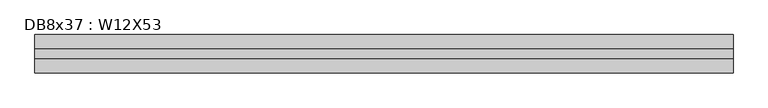
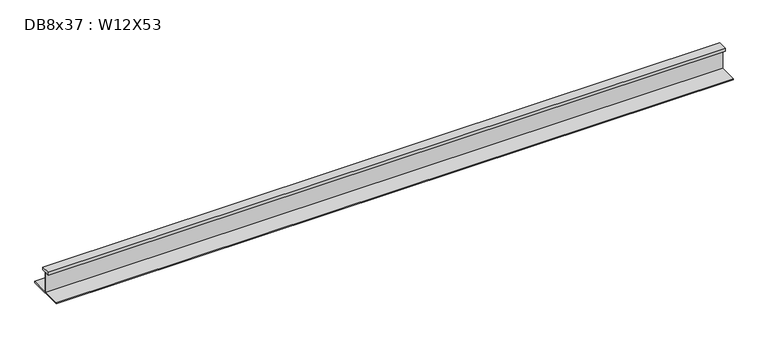
"""IFC4 building model written with IfcOpenShell, lengths in millimetres: beam geometry, DB8x37 : W12X53."""

import ifcopenshell
import ifcopenshell.guid

model = None  # the IFC model being written
_history = None  # IfcOwnerHistory: only IFC2X3 demands one
_inside = {}  # id of a spatial element -> (the spatial element, [elements in it])
_under = {}  # id of a project, library or spatial element -> (it, [spatial elements below it])
_declared = {}  # id of a project -> (the project, [libraries it declares])
_typed = {}  # id of a type object -> (the type object, [elements of that type])
_made_of = {}  # id of a material, layer set ... -> (it, [elements and type objects made of it])


def new_model(schema):
    """Start an empty IFC model of exactly this schema.

    Asked for "IFC4X3", IfcOpenShell would pick the latest addendum, in which some entities
    have other attributes; the version numbers below select the first issue.
    IFC2X3 requires an IfcOwnerHistory on every rooted entity: one is made here for all.
    """
    global model, _history
    if schema == "IFC4X3":
        model = ifcopenshell.file(schema_version=(4, 3, 0, 0))
    else:
        model = ifcopenshell.file(schema=schema)
    _inside.clear()
    _under.clear()
    _declared.clear()
    _typed.clear()
    _made_of.clear()
    _history = None
    if model.schema == "IFC2X3":
        org = make("IfcOrganization", Name="unknown")
        user = make(
            "IfcPersonAndOrganization",
            ThePerson=make("IfcPerson", FamilyName="unknown"),
            TheOrganization=org,
        )
        app = make(
            "IfcApplication",
            ApplicationDeveloper=org,
            Version="unknown",
            ApplicationFullName="unknown",
            ApplicationIdentifier="unknown",
        )
        _history = make(
            "IfcOwnerHistory",
            OwningUser=user,
            OwningApplication=app,
            ChangeAction="ADDED",
            CreationDate=0,
        )
    return model


def make(cls, **values):
    """One entity of the class cls with the attributes given. An attribute that is None is left unset."""
    return model.create_entity(
        cls, **{name: value for name, value in values.items() if value is not None}
    )


def rooted(cls, **values):
    """An entity with a GlobalId (a new one), such as an element, a storey or a relation."""
    return make(cls, GlobalId=ifcopenshell.guid.new(), OwnerHistory=_history, **values)


def si_unit(unit_type, name, prefix=None):
    """IfcSIUnit, for example si_unit("LENGTHUNIT", "METRE", prefix="MILLI")."""
    return make("IfcSIUnit", UnitType=unit_type, Prefix=prefix, Name=name)


def assignment(units):
    """IfcUnitAssignment: the units of a project."""
    return None if units is None else make("IfcUnitAssignment", Units=units)


def point(xyz):
    """IfcCartesianPoint."""
    return None if xyz is None else make("IfcCartesianPoint", Coordinates=xyz)


def direction(xyz):
    """IfcDirection."""
    return None if xyz is None else make("IfcDirection", DirectionRatios=xyz)


def frame(location, z_axis=None, x_axis=None):
    """IfcAxis2Placement3D, a coordinate frame: its origin and axes. An axis left out is left unset."""
    return make(
        "IfcAxis2Placement3D",
        Location=point(location),
        Axis=direction(z_axis),
        RefDirection=direction(x_axis),
    )


def origin():
    """The frame at (0, 0, 0) with its axes left unset."""
    return frame((0.0, 0.0, 0.0))


def place(relative_to, where):
    """IfcLocalPlacement: puts the frame where relative to a parent placement (None: the world)."""
    return make(
        "IfcLocalPlacement", PlacementRelTo=relative_to, RelativePlacement=where
    )


def context(
    kind, dimensions, precision=None, world=None, true_north=None, identifier=None
):
    """IfcGeometricRepresentationContext, for example the 3D "Model" context."""
    return make(
        "IfcGeometricRepresentationContext",
        ContextIdentifier=identifier,
        ContextType=kind,
        CoordinateSpaceDimension=dimensions,
        Precision=precision,
        WorldCoordinateSystem=world,
        TrueNorth=true_north,
    )


def project(units=None, contexts=None):
    """IfcProject with its units and contexts."""
    return rooted(
        "IfcProject",
        Name="project",
        RepresentationContexts=contexts,
        UnitsInContext=assignment(units),
    )


def spatial(cls, under=None, at=None, **own):
    """A site, building, storey or space (cls), placed at a placement, below another one or the project."""
    s = rooted(cls, ObjectPlacement=at, **own)
    if under is not None:
        _under.setdefault(under.id(), (under, []))[1].append(s)
    return s


def polyline(points):
    """IfcPolyline through the points."""
    return make("IfcPolyline", Points=[point(p) for p in points])


def outline(outer, holes=None, kind="AREA"):
    """IfcArbitraryClosedProfileDef: a profile drawn as a closed curve; with holes, ...WithVoids."""
    if holes is None:
        return make("IfcArbitraryClosedProfileDef", ProfileType=kind, OuterCurve=outer)
    return make(
        "IfcArbitraryProfileDefWithVoids",
        ProfileType=kind,
        OuterCurve=outer,
        InnerCurves=holes,
    )


def extrude(swept, where, along, depth):
    """IfcExtrudedAreaSolid: the profile swept, set in the frame where, extruded along a direction by depth."""
    return make(
        "IfcExtrudedAreaSolid",
        SweptArea=swept,
        Position=where,
        ExtrudedDirection=direction(along),
        Depth=depth,
    )


def shape(context_of_items, identifier, shape_type, items):
    """IfcShapeRepresentation: the items that make up one representation, for example the "Body"."""
    return make(
        "IfcShapeRepresentation",
        ContextOfItems=context_of_items,
        RepresentationIdentifier=identifier,
        RepresentationType=shape_type,
        Items=items,
    )


def source(mapping_origin, context_of_items, identifier, shape_type, items):
    """IfcRepresentationMap: a shape defined once, which mapped items show again and again."""
    return make(
        "IfcRepresentationMap",
        MappingOrigin=mapping_origin,
        MappedRepresentation=shape(context_of_items, identifier, shape_type, items),
    )


def transform(
    local_origin,
    x_axis=None,
    y_axis=None,
    z_axis=None,
    scale=None,
    scale2=None,
    scale3=None,
    uniform=True,
):
    """IfcCartesianTransformationOperator3D, or its non-uniform kind. x_axis, y_axis, z_axis: its Axis1, 2, 3."""
    if uniform:
        return make(
            "IfcCartesianTransformationOperator3D",
            Axis1=direction(x_axis),
            Axis2=direction(y_axis),
            LocalOrigin=point(local_origin),
            Scale=scale,
            Axis3=direction(z_axis),
        )
    return make(
        "IfcCartesianTransformationOperator3DnonUniform",
        Axis1=direction(x_axis),
        Axis2=direction(y_axis),
        LocalOrigin=point(local_origin),
        Scale=scale,
        Axis3=direction(z_axis),
        Scale2=scale2,
        Scale3=scale3,
    )


def mapped(mapping_source, mapping_target):
    """IfcMappedItem: shows the shape of a source again, moved by a transform."""
    return make(
        "IfcMappedItem", MappingSource=mapping_source, MappingTarget=mapping_target
    )


def made_of(thing, what):
    """Note that an element or type object is made of a material, layer set ...; save() writes the relation."""
    if what is not None:
        _made_of.setdefault(what.id(), (what, []))[1].append(thing)
    return thing


def element(
    cls,
    number,
    at=None,
    inside=None,
    cuts=None,
    type_object=None,
    material=None,
    context=None,
    identifier="Body",
    shape_type=None,
    held_by="IfcProductDefinitionShape",
    body=None,
    shapes=None,
    **own,
):
    """One element of the class cls, such as IfcWall. Its Tag is "e" and its number.

    at: its placement. inside: the storey or other place that contains it. cuts: it is an
    opening in that element (IfcRelVoidsElement). A single representation is given by context,
    identifier, shape_type and body (its items); several are given by shapes. held_by: the class
    of the entity that holds the representations. save() writes the other relations.
    """
    e = rooted(cls, Tag="e%d" % number, ObjectPlacement=at, **own)
    if body is not None:
        shapes = [shape(context, identifier, shape_type, body)]
    if shapes is not None:
        e.Representation = make(held_by, Representations=shapes)
    if inside is not None:
        _inside.setdefault(inside.id(), (inside, []))[1].append(e)
    if cuts is not None:
        rooted(
            "IfcRelVoidsElement", RelatingBuildingElement=cuts, RelatedOpeningElement=e
        )
    if type_object is not None:
        _typed.setdefault(type_object.id(), (type_object, []))[1].append(e)
    return made_of(e, material)


def aggregate(whole, parts):
    """IfcRelAggregates: a whole, such as a stair, and the parts it consists of."""
    return rooted("IfcRelAggregates", RelatingObject=whole, RelatedObjects=parts)


def save(model, path):
    """Write the relations noted so far, then the file.

    IfcRelAggregates (storeys below a building ...), IfcRelContainedInSpatialStructure (elements
    in a storey), IfcRelDefinesByType, IfcRelAssociatesMaterial and IfcRelDeclares: one each for
    every whole, place, type object, material and project.
    """
    for whole, parts in _under.values():
        aggregate(whole, parts)
    for where, things in _inside.values():
        rooted(
            "IfcRelContainedInSpatialStructure",
            RelatedElements=things,
            RelatingStructure=where,
        )
    for kind, things in _typed.values():
        rooted("IfcRelDefinesByType", RelatedObjects=things, RelatingType=kind)
    for what, things in _made_of.values():
        rooted("IfcRelAssociatesMaterial", RelatedObjects=things, RelatingMaterial=what)
    for by, libraries in _declared.values():
        rooted("IfcRelDeclares", RelatingContext=by, RelatedDefinitions=libraries)
    model.write(path)


def db8x37_w12x53_32b51aad(model_context):
    return source(origin(), model_context, "Body", "SweptSolid", [
        extrude(outline(polyline([(38.1, 145.415), (38.1, 120.015), (2.921, 120.015), (2.921, -48.4505), (152.4, -48.4505), (152.4, -58.1025), (-152.4, -58.1025), (-152.4, -48.4505), (-2.921, -48.4505), (-2.921, 120.015), (-38.1, 120.015), (-38.1, 145.415), (38.1, 145.415)])), frame((-2705.1, 0.0, 0.0), z_axis=(1.0, 0.0, 0.0), x_axis=(0.0, 1.0, 0.0)), (0.0, 0.0, 1.0), 5537.1999994),
    ])


if __name__ == "__main__":
    model = new_model("IFC4")
    model_context = context("Model", 3, world=origin())
    ifc_project = project(units=[si_unit("LENGTHUNIT", "METRE", prefix="MILLI")], contexts=[model_context])
    site = spatial("IfcSite", under=ifc_project)
    building = spatial("IfcBuilding", under=site)
    placement = place(None, origin())
    db8x37_w12x53_shape = db8x37_w12x53_32b51aad(model_context)
    element("IfcBeam", 1, ObjectType="DB8x37 : W12X53", at=placement, inside=building, context=model_context, shape_type="MappedRepresentation", body=[
        mapped(db8x37_w12x53_shape, transform((0.0, 0.0, 0.0), x_axis=(1.0, 0.0, 0.0), y_axis=(0.0, 1.0, 0.0), z_axis=(0.0, 0.0, 1.0))),
    ])
    save(model, "model.ifc")

# Revit data of these elements
# Type "DB8x37 : W12X53"
#   Assembly Code = "B10"
#   W = 53
#   Length [instance default] = 5' - 0"
#   bf = 0' - 10"
#   d = 1' - 0.1"
#   k = 0' - 1 3/8"
#   k2 = 0' - 0.8"
#   tf = 0' - 0.575"
#   tw = 0' - 0.345"
#   A = 0.108333 SF
#   Structural Material [instance default] = Steel ASTM A992
# Element 1 (IfcBeam, "DB8x37 : W12X53")
#   Materials on its faces: "Steel ASTM A992"
# Materials
#   "Steel ASTM A992": class "Metal", colour RGB 199 199 199, transparency 0, Description = "Structural steel 50ksi", Cost = 0
